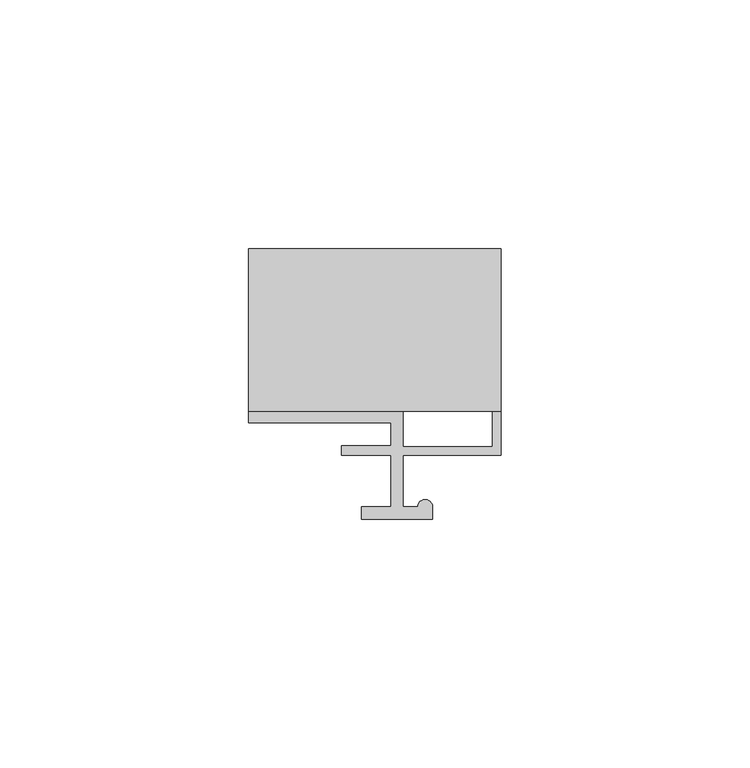
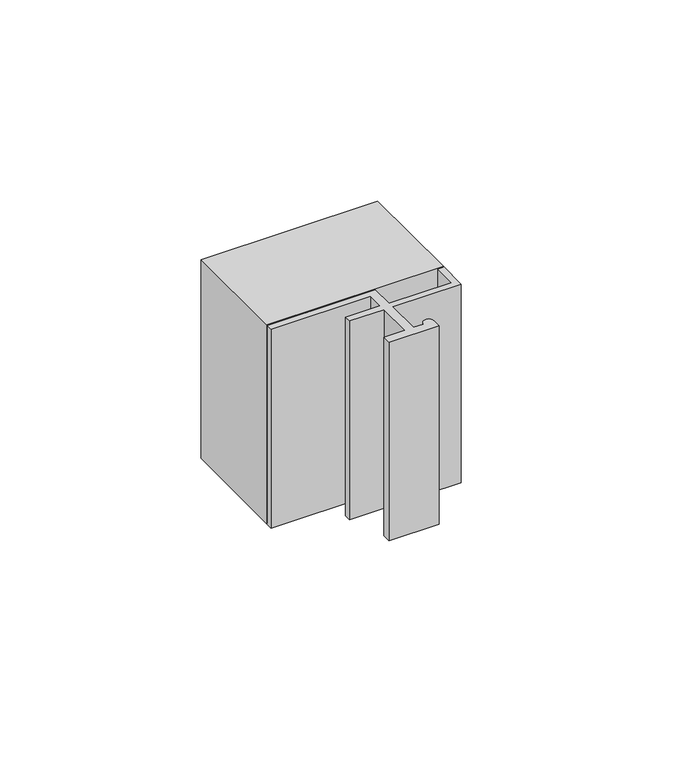
"""IFC4 building model written with IfcOpenShell, lengths in millimetres: proxy geometry, Generic Models 9:Generic Models 5:348123:Generic Models 5:348123 : Generic Models 9:Generic Models 5:348123:1 : Generic Models 9:Generic Models 5:348123:Generic Models 5:348123 : Generic Models 9:Generic Models 5:348123:301771."""

from ifc_helpers import new_model, si_unit, point, frame, frame_2d, origin, place, context, project, spatial, polyline, circle_curve, trimmed, segment, composite_curve, outline, extrude, source, transform, mapped, element, save


def generic_models_2b47b7e9(model_context):
    return source(origin(), model_context, "Body", "SweptSolid", [
        extrude(outline(polyline([(592204.7959377, -579000.6913841), (592255.5959377, -579000.6913841), (592255.5959377, -579033.3483921), (592204.7959377, -579033.3483921), (592204.7959377, -579000.6913841)])), frame((0.0, 0.0, 1233.0725209), z_axis=(0.0, 0.0, 1.0), x_axis=(1.0, 0.0, 0.0)), (0.0, 0.0, 1.0), 60.325),
        extrude(outline(composite_curve([segment(polyline([(592235.8677824, -579042.226062), (592235.8677824, -579052.5833435), (592238.8270057, -579052.5833435)]), True, "CONTINUOUS"), segment(trimmed(circle_curve(frame_2d((592240.3066173, -579052.5833435)), 1.4796117), [point((592238.8270057, -579052.5833435))], [point((592241.786229, -579052.5833435))], False, "CARTESIAN"), True, "CONTINUOUS"), segment(polyline([(592241.786229, -579052.5833435), (592241.786229, -579055.0493629), (592227.4833163, -579055.0493629), (592227.4833163, -579052.5833435), (592233.4017629, -579052.5833435), (592233.4017629, -579042.226062), (592223.5376853, -579042.226062), (592223.5376853, -579040.2532464), (592233.4017629, -579040.2532464), (592233.4017629, -579035.6171299), (592204.7959377, -579035.6171299), (592204.7959377, -579033.3483921), (592235.8677824, -579033.3483921), (592235.8677824, -579040.450528), (592253.8204037, -579040.450528), (592253.8204037, -579033.3483921), (592255.5959377, -579033.3483921), (592255.5959377, -579042.226062), (592235.8677824, -579042.226062)]), True, "CONTINUOUS")], self_intersect=False)), frame((0.0, 0.0, 1233.0725209), z_axis=(0.0, 0.0, 1.0), x_axis=(1.0, 0.0, 0.0)), (0.0, 0.0, 1.0), 60.325),
    ])


if __name__ == "__main__":
    model = new_model("IFC4")
    model_context = context("Model", 3, world=origin())
    ifc_project = project(units=[si_unit("LENGTHUNIT", "METRE", prefix="MILLI")], contexts=[model_context])
    site = spatial("IfcSite", under=ifc_project)
    building = spatial("IfcBuilding", under=site)
    placement = place(None, origin())
    generic_models_shape = generic_models_2b47b7e9(model_context)
    element("IfcBuildingElementProxy", 1, Name="Generic Models 9:Generic Models 5:348123:Generic Models 5:348123 : Generic Models 9:Generic Models 5:348123:1 : Generic Models 9:Generic Models 5:348123:Generic Models 5:348123 : Generic Models 9:Generic Models 5:348123:301771", ObjectType="Generic Models 9:Generic Models 5:348123:Generic Models 5:348123 : Generic Models 9:Generic Models 5:348123:1 : Generic Models 9:Generic Models 5:348123:Generic Models 5:348123 : Generic Models 9:Generic Models 5:348123:301771", at=placement, inside=building, context=model_context, shape_type="MappedRepresentation", body=[
        mapped(generic_models_shape, transform((0.0, 0.0, 0.0), x_axis=(1.0, 0.0, 0.0), y_axis=(0.0, 1.0, 0.0), z_axis=(0.0, 0.0, 1.0))),
    ])
    save(model, "model.ifc")

# Revit data of these elements
# Type "Generic Models 9:Generic Models 5:348123:Generic Models 5:348123 : Generic Models 9:Generic Models 5:348123:1 : Generic Models 9:Generic Models 5:348123:Generic Models 5:348123 : Generic Models 9:Generic Models 5:348123:301771"
#   NameOverride = "Generic Models 9:Generic Models 5:348123:Generic Models 5:348123 : Generic Models 9:Generic Models 5:348123:301771"
#   ObjectTypeOverride = "Generic Models 5:348123 : Generic Models 9:Generic Models 5:348123"
#   Reference = "Generic Models 5"
#   Tag = "301771"
# Element 1 (IfcBuildingElementProxy, "Generic Models 9:Generic Models 5:348123:Generic Models 5:348123 : Generic Models 9:Generic Models 5:348123:1 : Generic Models 9:Generic Models 5:348123:Generic Models 5:348123 : Generic Models 9:Generic Models 5:348123:301771")
#   Materials on its faces: "GA. STEEL CLIP AT EVERY SEAM IN POLYCARBONATE (WITH STEEL PLATE EXTENSION, IF NECS.)"
# Materials
#   "GA. STEEL CLIP AT EVERY SEAM IN POLYCARBONATE (WITH STEEL PLATE EXTENSION, IF NECS.)": class "Unassigned", colour RGB 120 120 120, transparency 0, Cost = 0
